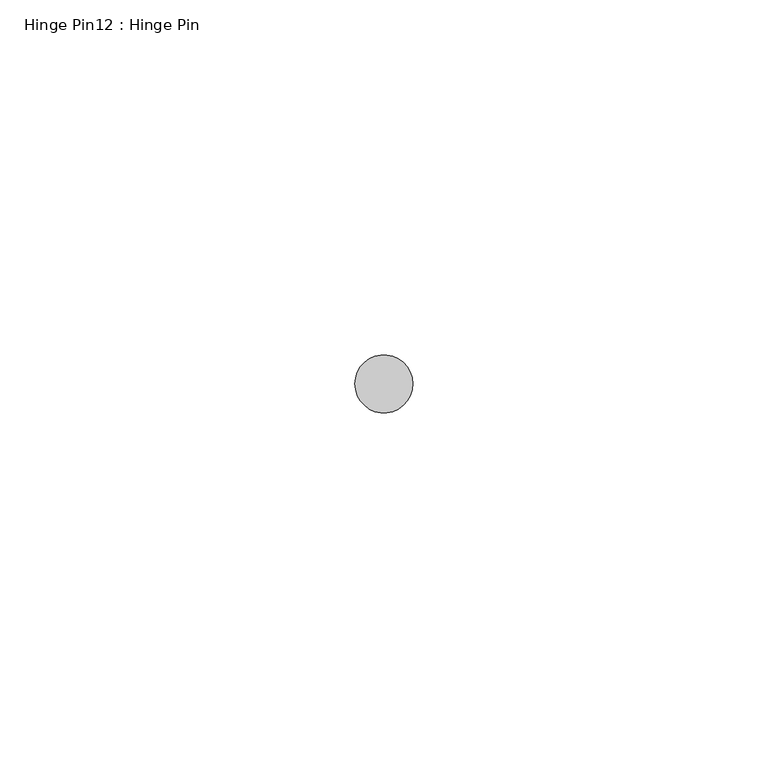
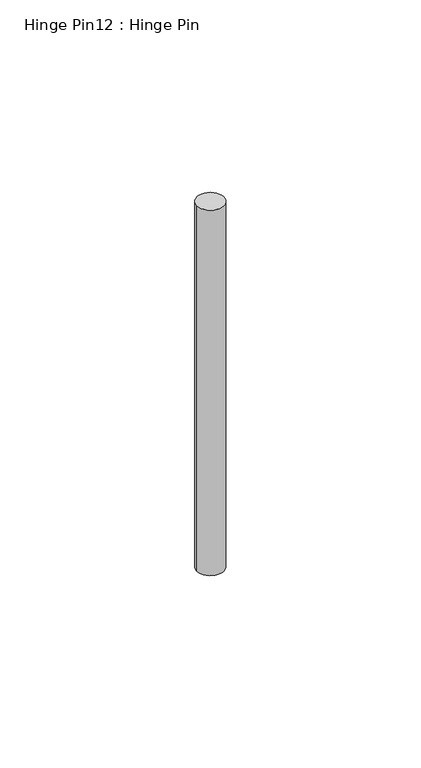
"""IFC4 building model written with IfcOpenShell, lengths in millimetres: proxy geometry, Hinge Pin12 : Hinge Pin."""

from ifc_helpers import new_model, si_unit, point, frame, frame_2d, origin, place, context, project, spatial, circle_curve, trimmed, segment, composite_curve, outline, extrude, source, transform, mapped, element, save


def hinge_pin12_hinge_pin_59ca42a9(model_context):
    return source(origin(), model_context, "Body", "SweptSolid", [
        extrude(outline(composite_curve([segment(trimmed(circle_curve(frame_2d((587319.1320739, -531776.6049841)), 4.0894), [point((587315.0426739, -531776.6049841))], [point((587323.2214739, -531776.6049841))], False, "CARTESIAN"), True, "CONTINUOUS"), segment(trimmed(circle_curve(frame_2d((587319.1320739, -531776.6049841)), 4.0894), [point((587323.2214739, -531776.6049841))], [point((587315.0426739, -531776.6049841))], False, "CARTESIAN"), True, "CONTINUOUS")], self_intersect=False)), frame((0.0, 0.0, 315.7140625), z_axis=(0.0, 0.0, 1.0), x_axis=(1.0, 0.0, 0.0)), (0.0, 0.0, 1.0), 117.871875),
    ])


if __name__ == "__main__":
    model = new_model("IFC4")
    model_context = context("Model", 3, world=origin())
    ifc_project = project(units=[si_unit("LENGTHUNIT", "METRE", prefix="MILLI")], contexts=[model_context])
    site = spatial("IfcSite", under=ifc_project)
    building = spatial("IfcBuilding", under=site)
    placement = place(None, origin())
    hinge_pin12_hinge_pin_shape = hinge_pin12_hinge_pin_59ca42a9(model_context)
    element("IfcBuildingElementProxy", 1, Name="Hinge Pin12 : Hinge Pin", ObjectType="Hinge Pin12 : Hinge Pin", at=placement, inside=building, context=model_context, shape_type="MappedRepresentation", body=[
        mapped(hinge_pin12_hinge_pin_shape, transform((0.0, 0.0, 0.0), x_axis=(1.0, 0.0, 0.0), y_axis=(0.0, 1.0, 0.0), z_axis=(0.0, 0.0, 1.0))),
    ])
    save(model, "model.ifc")

# Revit data of these elements
# Element 1 (IfcBuildingElementProxy, "Hinge Pin12 : Hinge Pin")
#   Materials on its faces: "6\"X6\" WELD-ON STL BUTT HINGE"
# Materials
#   "6\"X6\" WELD-ON STL BUTT HINGE": class "Metal", colour RGB 189 187 185, transparency 0, Description = "Carbon steel", Cost = 0
